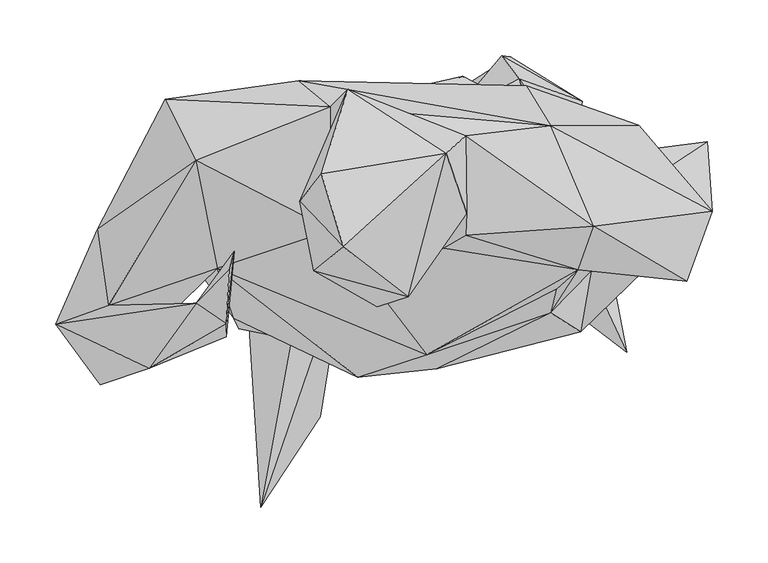
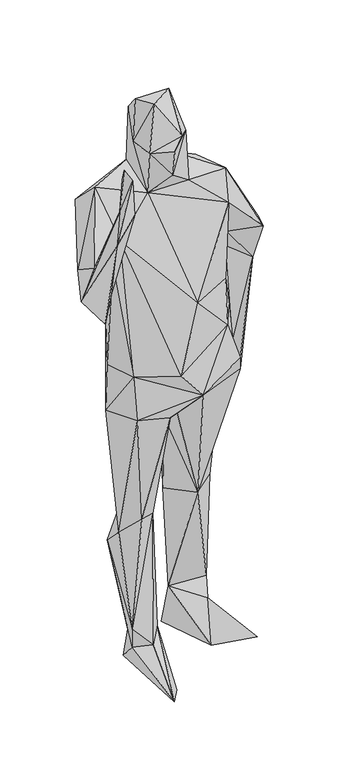
"""IFC4 building model written with IfcOpenShell, lengths in millimetres: geographic element geometry, Enscape AssetDefinition - Aadesh 003 Standing : Enscape AssetDefinition - Aadesh 003 Standing."""

from ifc_helpers import new_model, si_unit, origin, place, context, project, spatial, faceted_brep, source, transform, mapped, element, save


def geographic_element_f295e97e(model_context):
    return source(origin(), model_context, "Body", "Brep", [
        faceted_brep([(-116.0581186, 157.9167694, 799.051702), (-20.1751553, 76.9282728, 730.2228808), (-53.5155386, 80.2018344, 437.5201762), (19.4844585, 154.7251642, 446.2543726), (14.3677006, 160.7495397, 802.982986), (82.1649805, 81.7001835, 454.985559), (-18.5108855, 12.4965217, 782.5808525), (-69.4655478, -37.8534049, 816.2641525), (92.2375694, 202.1103948, 499.7079074), (76.6384006, 222.4984467, 164.9716794), (40.4422693, 161.4971906, 124.463439), (148.7198025, 181.7743033, 200.1702487), (84.0101689, 221.7098027, 79.8679888), (138.8731152, 117.0017123, 471.2873697), (141.3060427, 138.7421638, 136.2292767), (121.7826158, 99.3434414, 96.8185514), (153.1908363, 141.2360817, -2.0331086), (35.7983038, 190.7553822, -4.0962039), (144.2617476, 97.9240686, 642.7662373), (164.3969268, 3.5104612, 865.226686), (18.0400908, -58.6692803, 869.2498803), (149.3915021, 115.1895002, 851.4847159), (105.3678095, 159.6620083, 825.7749677), (41.4998084, 204.3294311, 942.3778653), (-173.440963, 116.8297827, 1063.6976957), (-108.4184647, 170.0184643, 1062.069416), (98.9146307, 173.9807278, 983.1470251), (-112.7445698, 135.2317184, 471.2633789), (-173.2340455, 48.9205532, 437.5601709), (-198.2760727, 73.329851, 818.4002042), (-112.9394844, 107.6528057, 74.1864741), (-175.9388745, 104.565151, 381.5637231), (-73.2958689, 100.6758586, 145.2033371), (-152.3042321, 13.8259381, 88.2143304), (-125.03618, 107.9806611, -5.1427456), (-70.962891, 113.4982407, 22.7680188), (-151.6065449, 15.460222, 142.8083926), (-139.8766786, -182.575956, 29.0482659), (-110.6964722, -23.0398998, 102.8439179), (-86.3441452, -101.3605669, 0.1809207), (-63.945964, 37.8534049, 110.4805693), (-127.2742003, 8.7251747, 487.205416), (-159.7409695, -22.5391183, 829.3944001), (-164.3119752, -13.2331988, 962.5620246), (120.4202101, -8.1204399, 1026.4759064), (147.640273, -25.3488868, 924.6606231), (-53.0007668, -66.0570413, 959.6602917), (157.1680903, 29.6120197, 942.2478676), (233.5026413, 58.0175631, 1161.4158154), (261.1085176, 145.1453716, 1155.9072733), (197.8302747, 137.3887658, 1161.939621), (242.855534, 19.8802836, 1279.9217701), (173.1081009, 87.2397572, 1246.4895248), (157.9907387, 50.1030311, 1041.9502258), (265.6635344, 83.0445886, 1262.7344131), (159.1062397, 69.4325641, 1463.7203217), (145.1473683, 30.0608221, 1383.2036257), (199.7804046, 160.1108164, 1344.8255062), (120.6680983, 159.4700962, 1464.8548365), (44.2326069, 61.3161214, 1470.7043171), (44.3515554, 150.7629007, 1505.6209564), (98.4118581, 195.4403222, 1210.8331919), (-105.6926697, 200.2112269, 1208.60219), (-77.4280578, 176.8434793, 1508.2108974), (175.524056, 148.1340528, 1277.5160074), (-8.368331, 174.5854616, 1055.8211803), (115.1645109, 161.5861654, 1063.0069971), (125.9947568, 13.1022558, 1160.2833271), (142.7494287, 68.4330016, 1166.1797762), (9.1739781, -46.0058302, 1157.7404737), (-76.6264051, 65.8291429, 1468.9459801), (-178.8146049, 31.7310877, 1372.8171587), (-200.0423074, 34.8327309, 1302.6409149), (-198.2940733, 65.8041537, 967.8387046), (-237.9916757, -25.562793, 1258.241415), (-207.3910683, 125.1971126, 1310.6224537), (-230.4109931, 64.3168092, 1268.6098814), (-225.5321294, 183.2606643, 1428.5657406), (-286.118567, 67.1275705, 1298.1379032), (-283.9215398, -72.8750527, 1209.4298601), (-198.4669864, 128.6635846, 1490.8974171), (-324.120909, -18.7597759, 1261.6369724), (-276.3318419, -1.6382819, 1340.5423164), (-239.8708463, -57.9925738, 1433.5844517), (-197.8372782, -0.0149934, 1491.0032749), (-61.620988, 192.5045997, 1660.3951454), (-104.9360037, 91.8477327, 1626.5569925), (-28.1756483, 19.4484722, 1534.7481966), (-92.3994929, 29.1372258, 1620.6015348), (45.2811457, 80.8335617, 1614.3232584), (-35.3964828, -3.0406669, 1625.8113384), (-7.4897166, 5.777467, 1660.6030464), (-65.8751205, 51.0156341, 1753.6520958), (26.6333241, 134.9748224, 1722.1499681), (-85.4365379, 116.2760258, 1739.1725779), (-170.9450483, -30.111799, 1489.1301394), (-163.5103226, 46.8364656, 1552.3124933), (-170.8731055, -18.4109285, 1591.355443), (-168.2972312, 30.0268363, 1593.8881636), (188.78223, -43.7258296, 35.4364626), (92.4664661, 30.187767, -1.7542311)], [[[0, 1, 2]], [[3, 1, 4]], [[1, 3, 5]], [[0, 4, 1]], [[1, 5, 6]], [[2, 1, 7]], [[1, 6, 7]], [[4, 8, 3]], [[3, 8, 9]], [[10, 5, 3]], [[3, 9, 10]], [[9, 8, 11]], [[12, 9, 11]], [[9, 12, 10]], [[11, 8, 13]], [[12, 11, 14]], [[11, 13, 14]], [[12, 15, 16]], [[14, 15, 12]], [[17, 10, 12]], [[12, 16, 17]], [[14, 5, 10]], [[5, 14, 13]], [[15, 14, 10]], [[13, 18, 5]], [[18, 13, 8]], [[5, 19, 20]], [[20, 6, 5]], [[19, 5, 18]], [[21, 19, 18]], [[8, 21, 18]], [[8, 22, 21]], [[22, 8, 4]], [[23, 21, 22]], [[23, 22, 4]], [[23, 4, 0]], [[24, 23, 0]], [[25, 23, 24]], [[23, 25, 26]], [[26, 21, 23]], [[0, 27, 28]], [[29, 24, 0]], [[0, 28, 29]], [[0, 2, 27]], [[27, 30, 31]], [[32, 27, 2]], [[31, 28, 27]], [[27, 32, 30]], [[33, 31, 30]], [[34, 33, 30]], [[30, 35, 34]], [[30, 32, 35]], [[33, 36, 31]], [[31, 36, 28]], [[33, 34, 37]], [[38, 33, 37]], [[33, 38, 36]], [[34, 39, 37]], [[34, 35, 39]], [[35, 40, 39]], [[40, 35, 32]], [[2, 40, 32]], [[38, 40, 2]], [[40, 38, 37]], [[39, 40, 37]], [[2, 36, 38]], [[36, 2, 41]], [[41, 28, 36]], [[42, 41, 7]], [[41, 2, 7]], [[28, 41, 42]], [[28, 42, 29]], [[42, 7, 20]], [[29, 42, 43]], [[42, 20, 43]], [[20, 7, 6]], [[44, 20, 45]], [[20, 44, 46]], [[46, 43, 20]], [[20, 19, 45]], [[47, 45, 48]], [[47, 44, 45]], [[45, 19, 48]], [[19, 49, 48]], [[47, 49, 19]], [[21, 47, 19]], [[47, 48, 50]], [[48, 51, 52]], [[49, 51, 48]], [[48, 52, 50]], [[49, 47, 50]], [[47, 53, 44]], [[21, 53, 47]], [[49, 54, 51]], [[50, 52, 49]], [[49, 52, 54]], [[55, 56, 51]], [[51, 56, 52]], [[51, 54, 55]], [[57, 58, 54]], [[54, 58, 55]], [[52, 57, 54]], [[55, 59, 56]], [[58, 60, 55]], [[55, 60, 59]], [[58, 61, 62]], [[61, 58, 57]], [[63, 58, 62]], [[63, 60, 58]], [[57, 64, 61]], [[64, 57, 52]], [[62, 61, 65]], [[61, 66, 65]], [[61, 64, 66]], [[66, 64, 52]], [[52, 56, 67]], [[68, 52, 67]], [[68, 66, 52]], [[53, 66, 68]], [[66, 53, 26]], [[26, 65, 66]], [[62, 65, 25]], [[65, 26, 25]], [[26, 53, 21]], [[53, 68, 67]], [[53, 67, 44]], [[56, 69, 67]], [[69, 44, 67]], [[44, 69, 46]], [[70, 71, 69]], [[70, 69, 56]], [[69, 71, 46]], [[43, 46, 71]], [[43, 72, 73]], [[43, 71, 72]], [[73, 29, 43]], [[24, 73, 72]], [[29, 73, 24]], [[72, 25, 24]], [[71, 74, 72]], [[25, 72, 75]], [[72, 76, 75]], [[74, 76, 72]], [[77, 62, 75]], [[77, 75, 76]], [[75, 62, 25]], [[78, 76, 79]], [[77, 76, 78]], [[76, 74, 79]], [[63, 62, 77]], [[78, 80, 77]], [[80, 63, 77]], [[79, 81, 78]], [[82, 80, 78]], [[81, 82, 78]], [[79, 83, 81]], [[79, 74, 83]], [[81, 84, 82]], [[83, 84, 81]], [[82, 84, 74]], [[71, 80, 82]], [[82, 74, 71]], [[71, 70, 80]], [[63, 80, 70]], [[70, 56, 59]], [[85, 70, 86]], [[70, 85, 63]], [[70, 59, 87]], [[70, 87, 88]], [[88, 86, 70]], [[87, 59, 89]], [[59, 60, 89]], [[90, 87, 89]], [[90, 88, 87]], [[88, 91, 92]], [[88, 90, 91]], [[88, 92, 86]], [[91, 90, 89]], [[89, 93, 91]], [[93, 89, 60]], [[93, 60, 85]], [[85, 60, 63]], [[93, 92, 91]], [[85, 94, 93]], [[93, 94, 92]], [[94, 86, 92]], [[94, 85, 86]], [[83, 74, 95]], [[84, 95, 74]], [[96, 95, 84]], [[97, 95, 96]], [[97, 83, 95]], [[84, 83, 97]], [[97, 98, 84]], [[98, 96, 84]], [[96, 98, 97]], [[99, 15, 100]], [[100, 15, 10]], [[99, 16, 15]], [[99, 100, 16]], [[17, 100, 10]], [[16, 100, 17]]]),
    ])


if __name__ == "__main__":
    model = new_model("IFC4")
    model_context = context("Model", 3, world=origin())
    ifc_project = project(units=[si_unit("LENGTHUNIT", "METRE", prefix="MILLI")], contexts=[model_context])
    site = spatial("IfcSite", under=ifc_project)
    building = spatial("IfcBuilding", under=site)
    placement = place(None, origin())
    geographic_element_shape = geographic_element_f295e97e(model_context)
    element("IfcGeographicElement", 1, ObjectType="Enscape AssetDefinition - Aadesh 003 Standing : Enscape AssetDefinition - Aadesh 003 Standing", at=placement, inside=building, context=model_context, shape_type="MappedRepresentation", body=[
        mapped(geographic_element_shape, transform((0.0, 0.0, 0.0), x_axis=(1.0, 0.0, 0.0), y_axis=(0.0, 1.0, 0.0), z_axis=(0.0, 0.0, 1.0))),
    ])
    save(model, "model.ifc")

# Revit data of these elements
# Type "Enscape AssetDefinition - Aadesh 003 Standing : Enscape AssetDefinition - Aadesh 003 Standing"
#   EnscapeAssetSource = "REMOTE"
#   EnscapeAssetId = "dd34d60d-27d6-4bc1-b528-ef20719276c7"
#   Height = 1753.652 mm
#   EnscapeNativeAssetHeight = 1753.652 mm
#   Default Elevation = 0
